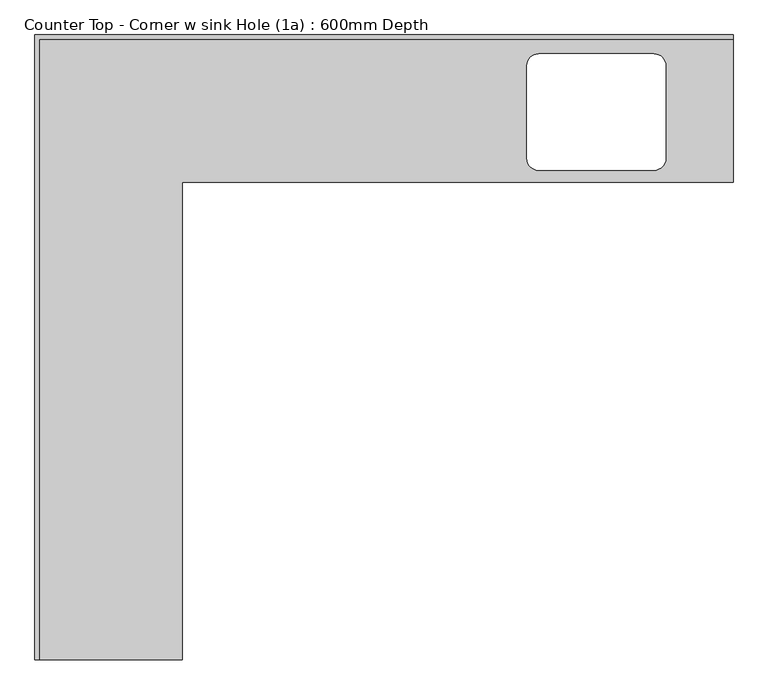
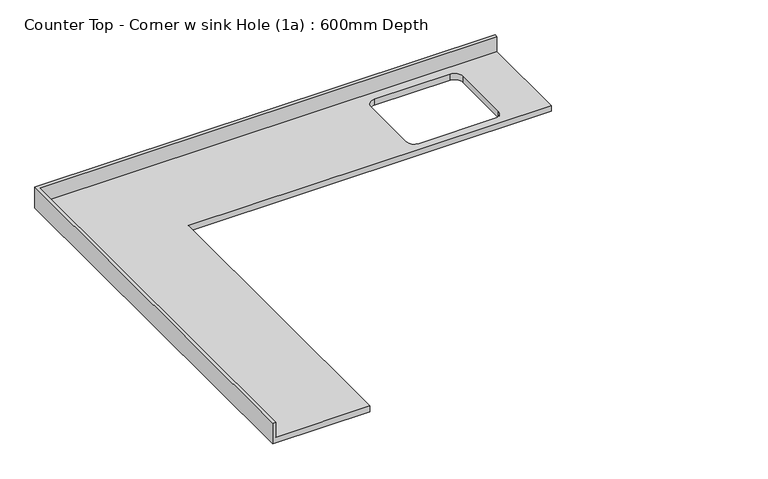
"""IFC4 building model written with IfcOpenShell, lengths in millimetres: furniture geometry, Counter Top - Corner w sink Hole (1a) : 600mm Depth."""

from ifc_helpers import new_model, si_unit, frame, origin, place, context, project, spatial, polyline, circle_curve, source, transform, mapped, element, save
from ifc_brep_helpers import plane_surface, revolved_surface, advanced_brep


def counter_top_corner_w_sink_hole_1a_600mm_depth_949058ad(model_context):
    return source(origin(), model_context, "Body", "AdvancedBrep", [
        advanced_brep(
        [(-575.4622951, -2650.0, 900.0), (-575.4622951, -625.0, 900.0), (1760.5377049, -625.0, 900.0), (1760.5377049, -19.05, 900.0), (-1181.4122951, -19.05, 900.0), (-1181.4122951, -2650.0, 900.0), (1424.9847176, -80.9334893, 900.0), (1474.9847176, -130.9334893, 900.0), (1474.9847176, -524.5706264, 900.0), (1424.9847176, -574.5706264, 900.0), (936.4146442, -574.5706264, 900.0), (886.4146442, -524.5706264, 900.0), (886.4146442, -130.9334893, 900.0), (936.4146442, -80.9334893, 900.0), (1760.5377049, 0.0, 860.0), (1760.5377049, -625.0, 860.0), (-575.4622951, -625.0, 860.0), (-575.4622951, -2650.0, 860.0), (-1200.4622951, -2650.0, 860.0), (-1200.4622951, 0.0, 860.0), (1424.9847176, -80.9334893, 860.0), (936.4146442, -80.9334893, 860.0), (886.4146442, -130.9334893, 860.0), (886.4146442, -524.5706264, 860.0), (936.4146442, -574.5706264, 860.0), (1424.9847176, -574.5706264, 860.0), (1474.9847176, -524.5706264, 860.0), (1474.9847176, -130.9334893, 860.0), (-1200.4622951, 0.0, 1001.6), (1760.5377049, 0.0, 1001.6), (-1200.4622951, -2650.0, 1001.6), (-1181.4122951, -2650.0, 1001.6), (1760.5377049, -19.05, 1001.6), (-1181.4122951, -19.05, 1001.6)],
        [
            (0, 1),
            (1, 2),
            (2, 3),
            (3, 4),
            (4, 5),
            (5, 0),
            (6, 7, circle_curve(frame((1424.9847176, -130.9334893, 900.0), z_axis=(0.0, 0.0, -1.0), x_axis=(1.0, 0.0, 0.0)), 50.0)),
            (7, 8),
            (8, 9, circle_curve(frame((1424.9847176, -524.5706264, 900.0), z_axis=(0.0, 0.0, -1.0), x_axis=(1.0, 0.0, 0.0)), 50.0)),
            (9, 10),
            (10, 11, circle_curve(frame((936.4146442, -524.5706264, 900.0), z_axis=(0.0, 0.0, -1.0), x_axis=(1.0, 0.0, 0.0)), 50.0)),
            (11, 12),
            (12, 13, circle_curve(frame((936.4146442, -130.9334893, 900.0), z_axis=(0.0, 0.0, -1.0), x_axis=(1.0, 0.0, 0.0)), 50.0)),
            (13, 6),
            (14, 15),
            (15, 16),
            (16, 17),
            (17, 18),
            (18, 19),
            (19, 14),
            (20, 21),
            (21, 22, circle_curve(frame((936.4146442, -130.9334893, 860.0), z_axis=(0.0, 0.0, 1.0), x_axis=(1.0, 0.0, 0.0)), 50.0)),
            (22, 23),
            (23, 24, circle_curve(frame((936.4146442, -524.5706264, 860.0), z_axis=(0.0, 0.0, 1.0), x_axis=(1.0, 0.0, 0.0)), 50.0)),
            (24, 25),
            (25, 26, circle_curve(frame((1424.9847176, -524.5706264, 860.0), z_axis=(0.0, 0.0, 1.0), x_axis=(1.0, 0.0, 0.0)), 50.0)),
            (26, 27),
            (27, 20, circle_curve(frame((1424.9847176, -130.9334893, 860.0), z_axis=(0.0, 0.0, 1.0), x_axis=(1.0, 0.0, 0.0)), 50.0)),
            (19, 28),
            (28, 29),
            (29, 14),
            (18, 30),
            (30, 28),
            (17, 0),
            (5, 31),
            (31, 30),
            (16, 1),
            (15, 2),
            (29, 32),
            (32, 3),
            (6, 20),
            (27, 7),
            (26, 8),
            (25, 9),
            (24, 10),
            (23, 11),
            (22, 12),
            (21, 13),
            (31, 33),
            (33, 32),
            (33, 4),
        ],
        [
            plane_surface(frame((-1200.4622951, 0.0, 900.0), z_axis=(0.0, 0.0, 1.0), x_axis=(-1.0, 0.0, 0.0))),
            plane_surface(frame((-1200.4622951, 0.0, 860.0), z_axis=(0.0, 0.0, -1.0), x_axis=(1.0, 0.0, 0.0))),
            plane_surface(frame((1760.5377049, 0.0, 900.0), z_axis=(0.0, 1.0, 0.0), x_axis=(0.0, 0.0, -1.0))),
            plane_surface(frame((-1200.4622951, 0.0, 900.0), z_axis=(-1.0, 0.0, 0.0), x_axis=(0.0, 0.0, -1.0))),
            plane_surface(frame((-1200.4622951, -2650.0, 900.0), z_axis=(0.0, -1.0, 0.0), x_axis=(0.0, 0.0, -1.0))),
            plane_surface(frame((-575.4622951, -2650.0, 900.0), z_axis=(1.0, 0.0, 0.0), x_axis=(0.0, 0.0, -1.0))),
            plane_surface(frame((-575.4622951, -625.0, 900.0), z_axis=(0.0, -1.0, 0.0), x_axis=(0.0, 0.0, -1.0))),
            plane_surface(frame((1760.5377049, -625.0, 900.0), z_axis=(1.0, 0.0, 0.0), x_axis=(0.0, 0.0, -1.0))),
            revolved_surface(polyline([(1474.9847176, -130.9334893, 860.0), (1474.9847176, -130.9334893, 900.0)]), (1424.9847176, -130.9334893, 0.0), (0.0, 0.0, -1.0)),
            plane_surface(frame((1474.9847176, -130.9334893, 900.0), z_axis=(-1.0, 0.0, 0.0), x_axis=(0.0, 0.0, -1.0))),
            revolved_surface(polyline([(1474.9847176, -524.5706264, 860.0), (1474.9847176, -524.5706264, 900.0)]), (1424.9847176, -524.5706264, 0.0), (0.0, 0.0, -1.0)),
            plane_surface(frame((1424.9847176, -574.5706264, 900.0), z_axis=(0.0, 1.0, 0.0), x_axis=(0.0, 0.0, -1.0))),
            revolved_surface(polyline([(986.4146442, -524.5706264, 860.0), (986.4146442, -524.5706264, 900.0)]), (936.4146442, -524.5706264, 0.0), (0.0, 0.0, -1.0)),
            plane_surface(frame((886.4146442, -524.5706264, 900.0), z_axis=(1.0, 0.0, 0.0), x_axis=(0.0, 0.0, -1.0))),
            revolved_surface(polyline([(986.4146442, -130.9334893, 860.0), (986.4146442, -130.9334893, 900.0)]), (936.4146442, -130.9334893, 0.0), (0.0, 0.0, -1.0)),
            plane_surface(frame((936.4146442, -80.9334893, 900.0), z_axis=(0.0, -1.0, 0.0), x_axis=(0.0, 0.0, -1.0))),
            plane_surface(frame((-1200.4622951, 0.0, 1001.6), z_axis=(0.0, 0.0, 1.0), x_axis=(0.0, -1.0, 0.0))),
            plane_surface(frame((-1200.4622951, -19.05, 1001.6), z_axis=(0.0, -1.0, 0.0), x_axis=(0.0, 0.0, -1.0))),
            plane_surface(frame((-1181.4122951, -2650.0, 1001.6), z_axis=(1.0, 0.0, 0.0), x_axis=(0.0, 0.0, -1.0))),
        ],
        [
            (0, [[1, 2, 3, 4, 5, 6], [7, 8, 9, 10, 11, 12, 13, 14]]),
            (1, [[15, 16, 17, 18, 19, 20], [21, 22, 23, 24, 25, 26, 27, 28]]),
            (2, [[-20, 29, 30, 31]]),
            (3, [[-19, 32, 33, -29]]),
            (4, [[-32, -18, 34, -6, 35, 36]]),
            (5, [[-1, -34, -17, 37]]),
            (6, [[-2, -37, -16, 38]]),
            (7, [[-15, -31, 39, 40, -3, -38]]),
            (8, [[-7, 41, -28, 42]]),
            (9, [[-8, -42, -27, 43]]),
            (10, [[-9, -43, -26, 44]]),
            (11, [[-10, -44, -25, 45]]),
            (12, [[-11, -45, -24, 46]]),
            (13, [[-12, -46, -23, 47]]),
            (14, [[-13, -47, -22, 48]]),
            (15, [[-14, -48, -21, -41]]),
            (16, [[-33, -36, 49, 50, -39, -30]]),
            (17, [[-40, -50, 51, -4]]),
            (18, [[-49, -35, -5, -51]]),
        ],
    ),
    ])


if __name__ == "__main__":
    model = new_model("IFC4")
    model_context = context("Model", 3, world=origin())
    ifc_project = project(units=[si_unit("LENGTHUNIT", "METRE", prefix="MILLI")], contexts=[model_context])
    site = spatial("IfcSite", under=ifc_project)
    building = spatial("IfcBuilding", under=site)
    placement = place(None, origin())
    counter_top_corner_w_sink_hole_1a_600mm_depth_shape = counter_top_corner_w_sink_hole_1a_600mm_depth_949058ad(model_context)
    element("IfcFurniture", 1, ObjectType="Counter Top - Corner w sink Hole (1a) : 600mm Depth", at=placement, inside=building, context=model_context, shape_type="MappedRepresentation", body=[
        mapped(counter_top_corner_w_sink_hole_1a_600mm_depth_shape, transform((0.0, 0.0, 0.0), x_axis=(1.0, 0.0, 0.0), y_axis=(0.0, 1.0, 0.0), z_axis=(0.0, 0.0, 1.0))),
    ])
    save(model, "model.ifc")

# Revit data of these elements
# Type "Counter Top - Corner w sink Hole (1a) : 600mm Depth"
#   Keynote = "N10"
#   Width = 625 mm
#   Counter Thickness = 40 mm
#   Depth = 625 mm
#   Height = 900 mm
#   Length - Leg 1 [instance default] = 2250 mm
#   Length - Leg 2 [instance default] = 2150 mm
#   Sink Location [instance default] = 1100 mm
#   Sink Location To Wall [instance default] = 150 mm
#   Sink Opening Depth [instance default] = 380 mm
#   Sink Opening Width [instance default] = 585 mm
#   Vis - Worktop Upstand = yes
#   Material Worktop = Laminate - Marble
# Element 1 (IfcFurniture, "Counter Top - Corner w sink Hole (1a) : 600mm Depth")
#   Length - Leg 1 = 2961 mm
#   Length - Leg 2 = 2650 mm
#   Sink Location = 2086.877 mm
#   Sink Location To Wall = 80.933 mm
#   Sink Opening Depth = 493.637 mm
#   Sink Opening Width = 588.57 mm
#   Materials on its faces: "Laminate - Marble"
# Materials
#   "Laminate - Marble": class "Miscellaneous", colour RGB 196 174 157, transparency 0
